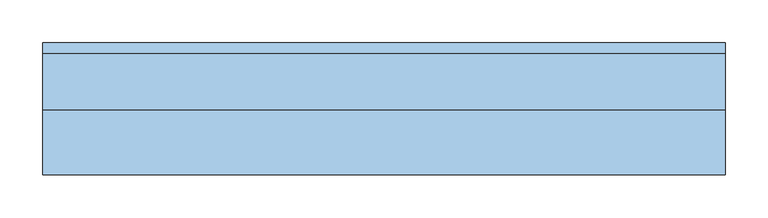
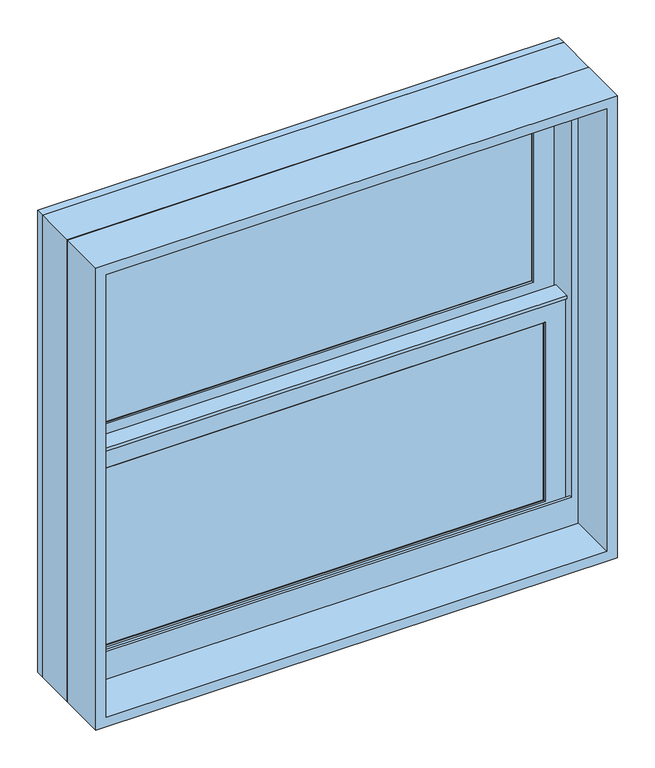
"""IFC4 building model written with IfcOpenShell, lengths in millimetres: window geometry, Window-Double_Hung-Marvin-Essential : ESDH2826."""

from ifc_helpers import new_model, si_unit, frame, origin, place, context, project, spatial, polyline, outline, extrude, faceted_brep, source, transform, mapped, element, save


def window_f95b2cba(model_context):
    return source(origin(), model_context, "Body", "SolidModel", [
        extrude(outline(polyline([(123.825, 20.6375), (123.825, 15.875), (104.775, 15.875), (104.775, 20.6375), (123.825, 20.6375)])), frame((0.0, 0.0, 1746.25), z_axis=(0.0, 0.0, 1.0), x_axis=(1.0, 0.0, 0.0)), (0.0, 0.0, 1.0), 298.45),
        extrude(outline(polyline([(-104.775, 20.6375), (-104.775, 15.875), (-123.825, 15.875), (-123.825, 20.6375), (-104.775, 20.6375)])), frame((0.0, 0.0, 1746.25), z_axis=(0.0, 0.0, 1.0), x_axis=(1.0, 0.0, 0.0)), (0.0, 0.0, 1.0), 298.45),
        extrude(outline(polyline([(342.9, 20.6375), (342.9, 15.875), (-342.9, 15.875), (-342.9, 20.6375), (342.9, 20.6375)])), frame((0.0, 0.0, 1885.95), z_axis=(0.0, 0.0, 1.0), x_axis=(1.0, 0.0, 0.0)), (0.0, 0.0, 1.0), 19.05),
        extrude(outline(polyline([(-123.825, 46.83125), (-123.825, 51.59375), (-104.775, 51.59375), (-104.775, 46.83125), (-123.825, 46.83125)])), frame((0.0, 0.0, 2082.8), z_axis=(0.0, 0.0, 1.0), x_axis=(1.0, 0.0, 0.0)), (0.0, 0.0, 1.0), 298.45),
        extrude(outline(polyline([(104.775, 46.83125), (104.775, 51.59375), (123.825, 51.59375), (123.825, 46.83125), (104.775, 46.83125)])), frame((0.0, 0.0, 2082.8), z_axis=(0.0, 0.0, 1.0), x_axis=(1.0, 0.0, 0.0)), (0.0, 0.0, 1.0), 298.45),
        extrude(outline(polyline([(-342.9, 46.83125), (-342.9, 51.59375), (342.9, 51.59375), (342.9, 46.83125), (-342.9, 46.83125)])), frame((0.0, 0.0, 2222.5), z_axis=(0.0, 0.0, 1.0), x_axis=(1.0, 0.0, 0.0)), (0.0, 0.0, 1.0), 19.05),
        extrude(outline(polyline([(123.825, 20.6375), (104.775, 20.6375), (104.775, 25.4), (123.825, 25.4), (123.825, 20.6375)])), frame((0.0, 0.0, 1746.25), z_axis=(0.0, 0.0, 1.0), x_axis=(1.0, 0.0, 0.0)), (0.0, 0.0, 1.0), 298.45),
        extrude(outline(polyline([(-104.775, 20.6375), (-123.825, 20.6375), (-123.825, 25.4), (-104.775, 25.4), (-104.775, 20.6375)])), frame((0.0, 0.0, 1746.25), z_axis=(0.0, 0.0, 1.0), x_axis=(1.0, 0.0, 0.0)), (0.0, 0.0, 1.0), 298.45),
        extrude(outline(polyline([(342.9, 20.6375), (-342.9, 20.6375), (-342.9, 25.4), (342.9, 25.4), (342.9, 20.6375)])), frame((0.0, 0.0, 1885.95), z_axis=(0.0, 0.0, 1.0), x_axis=(1.0, 0.0, 0.0)), (0.0, 0.0, 1.0), 19.05),
        extrude(outline(polyline([(-123.825, 56.35625), (-104.775, 56.35625), (-104.775, 51.59375), (-123.825, 51.59375), (-123.825, 56.35625)])), frame((0.0, 0.0, 2082.8), z_axis=(0.0, 0.0, 1.0), x_axis=(1.0, 0.0, 0.0)), (0.0, 0.0, 1.0), 298.45),
        extrude(outline(polyline([(104.775, 56.35625), (123.825, 56.35625), (123.825, 51.59375), (104.775, 51.59375), (104.775, 56.35625)])), frame((0.0, 0.0, 2082.8), z_axis=(0.0, 0.0, 1.0), x_axis=(1.0, 0.0, 0.0)), (0.0, 0.0, 1.0), 298.45),
        extrude(outline(polyline([(-342.9, 56.35625), (342.9, 56.35625), (342.9, 51.59375), (-342.9, 51.59375), (-342.9, 56.35625)])), frame((0.0, 0.0, 2222.5), z_axis=(0.0, 0.0, 1.0), x_axis=(1.0, 0.0, 0.0)), (0.0, 0.0, 1.0), 19.05),
        faceted_brep([(-369.8875, 5.6780605, 2074.7351748), (-369.8875, 5.6780605, 2070.1), (369.8875, 5.6780605, 2070.1), (369.8875, 5.6780605, 2074.7351748), (-369.8875, 34.8118605, 2074.7351748), (369.8875, 34.8118605, 2074.7351748), (369.8875, 34.8118605, 2070.1), (-369.8875, 34.8118605, 2070.1), (-369.8875, 30.1625, 2070.1), (-369.8875, 30.1625, 1719.2625), (-369.8875, 8.9241104, 1719.2625), (-369.8875, 8.9241104, 2070.1), (369.8875, 8.9241104, 2070.1), (369.8875, 30.1625, 2070.1), (369.8875, 8.9241104, 1719.2625), (369.8875, 30.1625, 1719.2625), (-354.0034752, 11.90625, 2055.8034752), (-354.0034752, 30.1625, 2055.8034752), (354.0034752, 30.1625, 2055.8034752), (354.0034752, 11.90625, 2055.8034752), (-337.34375, 10.4662439, 2039.14375), (-337.34375, 11.90625, 2039.14375), (337.34375, 11.90625, 2039.14375), (337.34375, 10.4662439, 2039.14375), (338.8858834, 8.9241104, 2040.6858834), (-338.8858834, 8.9241104, 2040.6858834), (354.0034752, 30.1625, 1735.1465248), (354.0034752, 11.90625, 1735.1465248), (337.34375, 11.90625, 1751.80625), (337.34375, 10.4662439, 1751.80625), (338.8858834, 8.9241104, 1750.2641166), (-354.0034752, 30.1625, 1735.1465248), (-354.0034752, 11.90625, 1735.1465248), (-337.34375, 11.90625, 1751.80625), (-337.34375, 10.4662439, 1751.80625), (-338.8858834, 8.9241104, 1750.2641166)], [[[0, 1, 2, 3]], [[4, 5, 6, 7]], [[1, 0, 4, 7, 8, 9, 10, 11]], [[2, 1, 11, 12]], [[7, 6, 13, 8]], [[3, 2, 12, 14, 15, 13, 6, 5]], [[0, 3, 5, 4]], [[16, 17, 18, 19]], [[20, 21, 22, 23]], [[20, 23, 24, 25]], [[19, 18, 26, 27]], [[23, 22, 28, 29]], [[24, 23, 29, 30]], [[27, 26, 31, 32]], [[29, 28, 33, 34]], [[30, 29, 34, 35]], [[15, 14, 10, 9]], [[15, 9, 8, 13], [18, 17, 31, 26]], [[17, 16, 32, 31]], [[16, 19, 27, 32], [22, 21, 33, 28]], [[21, 20, 34, 33]], [[20, 25, 35, 34]], [[10, 14, 12, 11], [25, 24, 30, 35]]]),
        extrude(outline(polyline([(38.5955581, 2055.8125), (33.5778968, 2055.8125), (33.5778968, 2057.4), (39.9405976, 2057.4), (39.9405976, 2055.8125), (61.515625, 2055.8125), (47.6307501, 2052.4975159), (38.5955581, 2052.4975159), (38.5955581, 2055.8125)])), frame((-369.8875, 0.0, 0.0), z_axis=(1.0, 0.0, 0.0), x_axis=(0.0, 1.0, 0.0)), (0.0, 0.0, 1.0), 739.775),
        faceted_brep([(400.05, 0.0, 1689.1), (400.05, 0.0, 2438.4), (-400.05, 0.0, 2438.4), (-400.05, 0.0, 1689.1), (373.85625, 0.0, 1750.21875), (-373.85625, 0.0, 1750.21875), (-373.85625, 0.0, 2412.20625), (373.85625, 0.0, 2412.20625), (373.85625, 3.96875, 1689.1), (-373.85625, 3.96875, 1689.1), (-373.85625, 3.96875, 1750.21875), (373.85625, 3.96875, 1750.21875), (-400.05, 65.6828125, 1689.1), (-373.85625, 65.6828125, 1689.1), (373.85625, 65.6828125, 1689.1), (400.05, 65.6828125, 1689.1), (-400.05, 65.6828125, 2438.4), (400.05, 65.6828125, 2438.4), (373.85625, 65.6828125, 2412.20625), (-373.85625, 65.6828125, 2412.20625)], [[[0, 1, 2, 3], [4, 5, 6, 7]], [[8, 9, 10, 11]], [[5, 4, 11, 10]], [[0, 3, 12, 13, 9, 8, 14, 15]], [[13, 12, 16, 17, 15, 14, 18, 19]], [[13, 19, 6, 5, 10, 9]], [[7, 6, 19, 18]], [[18, 14, 8, 11, 4, 7]], [[1, 0, 15, 17]], [[2, 1, 17, 16]], [[3, 2, 16, 12]]]),
        faceted_brep([(373.85625, 30.1625, 2063.75), (372.26875, 30.1625, 2063.75), (372.26875, 30.1625, 1713.4544613), (373.85625, 30.1625, 1713.4544613), (-372.26875, 30.1625, 2063.75), (-373.85625, 30.1625, 2063.75), (-373.85625, 30.1625, 1713.4544613), (-372.26875, 30.1625, 1713.4544613), (372.26875, 63.5, 2063.75), (373.85625, 63.5, 2063.75), (373.85625, 63.5, 1706.9743077), (372.26875, 63.5, 1706.9743077), (-373.85625, 63.5, 2063.75), (-372.26875, 63.5, 2063.75), (-372.26875, 63.5, 1706.9743077), (-373.85625, 63.5, 1706.9743077), (385.1108932, 3.96875, 1718.5460105), (385.1108932, 3.96875, 1689.1), (385.1108932, 65.6828125, 1689.1), (385.1108932, 65.6828125, 1706.550012), (-385.1108932, 3.96875, 1689.1), (-385.1108932, 3.96875, 1718.5460105), (-385.1108932, 65.6828125, 1706.550012), (-385.1108932, 65.6828125, 1689.1), (385.1108932, 78.58125, 1704.0428097), (-385.1108932, 78.58125, 1704.0428097), (-383.0971252, 68.2348864, 1706.0539391), (-365.13135, 68.2348864, 1706.0539391), (-365.13135, 65.6828125, 1706.550012), (365.13135, 65.6828125, 1706.550012), (365.13135, 68.2348864, 1706.0539391), (383.0971252, 68.2348864, 1706.0539391), (-400.05, 65.6828125, 1689.1), (-400.05, 78.5948249, 1689.1), (400.05, 78.5948249, 1689.1), (400.05, 65.6828125, 1689.1), (-400.05, 78.58125, 2438.4), (400.05, 78.58125, 2438.4), (385.1108932, 78.58125, 2423.4608932), (-385.1108932, 78.58125, 2423.4608932), (-400.05, 65.6828125, 2438.4), (-383.0971252, 68.2348864, 2421.4471252), (383.0971252, 68.2348864, 2421.4471252), (365.13135, 68.2348864, 2403.48135), (-365.13135, 68.2348864, 2403.48135), (-365.13135, 65.6828125, 2403.48135), (365.13135, 65.6828125, 2403.48135), (400.05, 65.6828125, 2438.4)], [[[0, 1, 2, 3]], [[4, 5, 6, 7]], [[8, 9, 10, 11]], [[12, 13, 14, 15]], [[1, 8, 11, 2]], [[9, 0, 3, 10]], [[1, 0, 9, 8]], [[5, 4, 13, 12]], [[5, 12, 15, 6]], [[13, 4, 7, 14]], [[16, 17, 18, 19]], [[20, 21, 22, 23]], [[24, 25, 26, 27, 28, 22, 21, 16, 19, 29, 30, 31], [3, 2, 11, 10], [7, 6, 15, 14]], [[17, 16, 21, 20]], [[17, 20, 23, 32, 33, 34, 35, 18]], [[34, 33, 36, 37], [25, 24, 38, 39]], [[33, 32, 40, 36]], [[39, 41, 26, 25]], [[41, 42, 31, 30, 43, 44, 27, 26]], [[44, 45, 28, 27]], [[40, 32, 23, 22, 28, 45, 46, 29, 19, 18, 35, 47]], [[36, 40, 47, 37]], [[39, 38, 42, 41]], [[44, 43, 46, 45]], [[34, 37, 47, 35]], [[42, 38, 24, 31]], [[46, 43, 30, 29]]]),
        extrude(outline(polyline([(350.04375, 11.90625), (-350.04375, 11.90625), (-350.04375, 15.08125), (350.04375, 15.08125), (350.04375, 11.90625)])), frame((0.0, 0.0, 1739.10625), z_axis=(0.0, 0.0, 1.0), x_axis=(1.0, 0.0, 0.0)), (0.0, 0.0, 1.0), 312.7375),
        extrude(outline(polyline([(350.04375, 42.8625), (-350.04375, 42.8625), (-350.04375, 46.0375), (350.04375, 46.0375), (350.04375, 42.8625)])), frame((0.0, 0.0, 2075.65625), z_axis=(0.0, 0.0, 1.0), x_axis=(1.0, 0.0, 0.0)), (0.0, 0.0, 1.0), 312.7375),
        faceted_brep([(-337.34375, 31.194477, 2039.14375), (-338.8858834, 32.7366104, 2040.6858834), (338.8858834, 32.7366104, 2040.6858834), (337.34375, 31.194477, 2039.14375), (-337.34375, 30.1625, 2039.14375), (337.34375, 30.1625, 2039.14375), (-369.8875, 32.7366104, 2071.6875), (-369.8875, 30.1625, 2071.6875), (369.8875, 30.1625, 2071.6875), (369.8875, 32.7366104, 2071.6875), (338.8858834, 32.7366104, 1750.2641166), (337.34375, 31.194477, 1751.80625), (337.34375, 30.1625, 1751.80625), (369.8875, 30.1625, 1719.2625), (369.8875, 32.7366104, 1719.2625), (-338.8858834, 32.7366104, 1750.2641166), (-337.34375, 31.194477, 1751.80625), (-337.34375, 30.1625, 1751.80625), (-369.8875, 30.1625, 1719.2625), (-369.8875, 32.7366104, 1719.2625)], [[[0, 1, 2, 3]], [[4, 0, 3, 5]], [[6, 7, 8, 9]], [[3, 2, 10, 11]], [[5, 3, 11, 12]], [[9, 8, 13, 14]], [[11, 10, 15, 16]], [[12, 11, 16, 17]], [[14, 13, 18, 19]], [[9, 14, 19, 6], [1, 15, 10, 2]], [[16, 15, 1, 0]], [[17, 16, 0, 4]], [[7, 18, 13, 8], [5, 12, 17, 4]], [[19, 18, 7, 6]]]),
        faceted_brep([(-354.0034752, 42.8625, 2392.3534752), (-354.0034752, 61.11875, 2392.3534752), (354.0034752, 61.11875, 2392.3534752), (354.0034752, 42.8625, 2392.3534752), (-337.34375, 41.4224939, 2375.69375), (-337.34375, 42.8625, 2375.69375), (337.34375, 42.8625, 2375.69375), (337.34375, 41.4224939, 2375.69375), (-338.8858834, 39.8803604, 2377.2358834), (338.8858834, 39.8803604, 2377.2358834), (-369.8875, 61.11875, 2408.2375), (-369.8875, 39.8803604, 2408.2375), (369.8875, 39.8803604, 2408.2375), (369.8875, 61.11875, 2408.2375), (354.0034752, 61.11875, 2071.6965248), (354.0034752, 42.8625, 2071.6965248), (337.34375, 42.8625, 2088.35625), (337.34375, 41.4224939, 2088.35625), (338.8858834, 39.8803604, 2086.8141166), (369.8875, 39.8803604, 2055.8125), (369.8875, 61.11875, 2055.8125), (-354.0034752, 61.11875, 2071.6965248), (-354.0034752, 42.8625, 2071.6965248), (-337.34375, 42.8625, 2088.35625), (-337.34375, 41.4224939, 2088.35625), (-338.8858834, 39.8803604, 2086.8141166), (-369.8875, 39.8803604, 2055.8125), (-369.8875, 61.11875, 2055.8125)], [[[0, 1, 2, 3]], [[4, 5, 6, 7]], [[8, 4, 7, 9]], [[10, 11, 12, 13]], [[3, 2, 14, 15]], [[7, 6, 16, 17]], [[9, 7, 17, 18]], [[13, 12, 19, 20]], [[15, 14, 21, 22]], [[17, 16, 23, 24]], [[18, 17, 24, 25]], [[20, 19, 26, 27]], [[13, 20, 27, 10], [1, 21, 14, 2]], [[22, 21, 1, 0]], [[3, 15, 22, 0], [5, 23, 16, 6]], [[24, 23, 5, 4]], [[25, 24, 4, 8]], [[11, 26, 19, 12], [9, 18, 25, 8]], [[27, 26, 11, 10]]]),
        faceted_brep([(-369.8875, 61.11875, 2055.8125), (-369.8875, 63.6928604, 2055.8125), (369.8875, 63.6928604, 2055.8125), (369.8875, 61.11875, 2055.8125), (-337.34375, 62.150727, 2088.35625), (-337.34375, 61.11875, 2088.35625), (337.34375, 61.11875, 2088.35625), (337.34375, 62.150727, 2088.35625), (-338.8858834, 63.6928604, 2086.8141166), (338.8858834, 63.6928604, 2086.8141166), (369.8875, 63.6928604, 2408.2375), (369.8875, 61.11875, 2408.2375), (337.34375, 61.11875, 2375.69375), (337.34375, 62.150727, 2375.69375), (338.8858834, 63.6928604, 2377.2358834), (-369.8875, 63.6928604, 2408.2375), (-369.8875, 61.11875, 2408.2375), (-337.34375, 61.11875, 2375.69375), (-337.34375, 62.150727, 2375.69375), (-338.8858834, 63.6928604, 2377.2358834)], [[[0, 1, 2, 3]], [[4, 5, 6, 7]], [[8, 4, 7, 9]], [[3, 2, 10, 11]], [[7, 6, 12, 13]], [[9, 7, 13, 14]], [[11, 10, 15, 16]], [[13, 12, 17, 18]], [[14, 13, 18, 19]], [[16, 15, 1, 0]], [[3, 11, 16, 0], [5, 17, 12, 6]], [[18, 17, 5, 4]], [[19, 18, 4, 8]], [[1, 15, 10, 2], [9, 14, 19, 8]]]),
        extrude(outline(polyline([(350.04375, 26.19375), (-350.04375, 26.19375), (-350.04375, 30.1625), (350.04375, 30.1625), (350.04375, 26.19375)])), frame((0.0, 0.0, 1739.10625), z_axis=(0.0, 0.0, 1.0), x_axis=(1.0, 0.0, 0.0)), (0.0, 0.0, 1.0), 312.7375),
        extrude(outline(polyline([(350.04375, 57.15), (-350.04375, 57.15), (-350.04375, 61.11875), (350.04375, 61.11875), (350.04375, 57.15)])), frame((0.0, 0.0, 2075.65625), z_axis=(0.0, 0.0, 1.0), x_axis=(1.0, 0.0, 0.0)), (0.0, 0.0, 1.0), 312.7375),
        extrude(outline(polyline([(2438.4, 400.05), (2438.4, -400.05), (1689.1, -400.05), (1689.1, 400.05), (2438.4, 400.05)]), holes=[polyline([(2422.525, 384.175), (1704.975, 384.175), (1704.975, -384.175), (2422.525, -384.175), (2422.525, 384.175)])]), frame((0.0, -76.2, 0.0), z_axis=(0.0, 1.0, 0.0), x_axis=(0.0, 0.0, 1.0)), (0.0, 0.0, 1.0), 75.40625),
    ])


if __name__ == "__main__":
    model = new_model("IFC4")
    model_context = context("Model", 3, world=origin())
    ifc_project = project(units=[si_unit("LENGTHUNIT", "METRE", prefix="MILLI")], contexts=[model_context])
    site = spatial("IfcSite", under=ifc_project)
    building = spatial("IfcBuilding", under=site)
    placement = place(None, origin())
    window_shape = window_f95b2cba(model_context)
    element("IfcWindow", 1, ObjectType="Window-Double_Hung-Marvin-Essential : ESDH2826", at=placement, inside=building, context=model_context, shape_type="MappedRepresentation", body=[
        mapped(window_shape, transform((0.0, 0.0, 0.0), x_axis=(1.0, 0.0, 0.0), y_axis=(0.0, 1.0, 0.0), z_axis=(0.0, 0.0, 1.0))),
    ])
    save(model, "model.ifc")

# Revit data of these elements
# Type "Window-Double_Hung-Marvin-Essential : ESDH2826"
#   Type Mark = "29"
#   Window Type = "Essential Double Hung"
#   Product data url = "https://bimobject.com/marvin-windows-and-doors/product/marvin-dhwau"
#   Product Guid = "c4a96547-874c-4385-91dc-a058adc19d98"
#   Frame = "All Ultrex"
#   Egress Window = "No"
#   URL = "www.marvin.com"
#   Model = "ESDH2826"
#   Manufacturer = "Marvin Windows and Doors"
#   Label Egress = ""
#   Glass Type = "IG Low E II with Argon"
#   Design Pressure = "DP50"
#   Description = "3230 DBHG"
#   Analytic Construction = "<None>"
#   Prairie Corner Width = 0' - 4"
#   Prairie Corner Height = 0' - 4"
#   Egress Width = 2' - 4 9/16"
#   Egress Height = 0' - 10 27/128"
#   Rough Width = 2' - 8"
#   Rough Height = 2' - 6"
#   Nominal Width = 2' - 8"
#   Nominal Height = 2' - 6"
#   Inset to Installation Flange [instance default] = 0' - 1"
#   Height = 2' - 5 1/2"
#   Egress Area = 2.02535 SF
#   Default Head Height = 8' - 0"
#   Width = 2' - 7 1/2"
#   Daylight Area = 4.17345 SF
#   DLO Width = 2' - 2 9/16"
#   DLO Height = 0' - 11 5/16"
#   Muntins Top Sash = yes
#   Lites Wide Top Sash = 3
#   Lites Wide Bottom Sash = 3
#   Lites High Top Sash = 2
#   Lites High Bottom Sash = 2
#   Lite Cut Prairie 9 = no
#   Lite Cut HV Grid = yes
#   Muntins Bottom Sash = yes
#   Label Visibility = no
#   Jamb Extension Visibility = yes
#   Edition number = 1
#   Interior Material = Ultrex-Marvin-Stonewhite
#   Glazing Material = Glass-Marvin-IG Low E II with Argon
#   Cladding Material = Ultrex-Marvin-Pebblegray
#   Wall Closure = (empty or 0)
#   Assembly Code = ""
# Element 1 (IfcWindow, "Window-Double_Hung-Marvin-Essential : ESDH2826")
#   Materials on its faces: "Ultrex-Marvin-Pebblegray", "Ultrex-Marvin-Stonewhite", "Glass-Marvin-IG Low E II with Argon"
# Materials
#   "Ultrex-Marvin-Stonewhite": class "Paint", colour RGB 250 251 245, transparency 0
#   "Glass-Marvin-IG Low E II with Argon": class "Glass", colour RGB 0 128 192, transparency 0.85
#   "Ultrex-Marvin-Pebblegray": class "Paint", colour RGB 189 185 173, transparency 0
